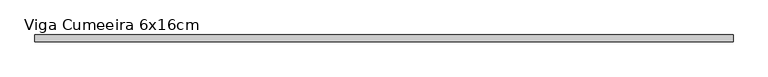
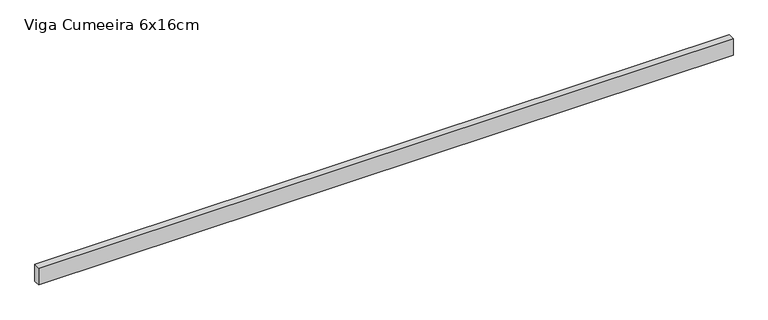
"""IFC4 building model written with IfcOpenShell, lengths in millimetres: beam geometry, Madeira de lei : Viga Cumeeira 6x16cm."""

from ifc_helpers import new_model, si_unit, frame, origin, place, context, project, spatial, polyline, outline, extrude, source, transform, mapped, element, save


def viga_cumeeira_6x16cm_e360fa9d(model_context):
    return source(origin(), model_context, "Body", "SweptSolid", [
        extrude(outline(polyline([(3133.5, 30.0), (3133.5, -30.0), (-3133.5, -30.0), (-3133.5, 30.0), (3133.5, 30.0)])), frame((0.0, 0.0, -80.0), z_axis=(0.0, 0.0, 1.0), x_axis=(1.0, 0.0, 0.0)), (0.0, 0.0, 1.0), 160.0),
    ])


if __name__ == "__main__":
    model = new_model("IFC4")
    model_context = context("Model", 3, world=origin())
    ifc_project = project(units=[si_unit("LENGTHUNIT", "METRE", prefix="MILLI")], contexts=[model_context])
    site = spatial("IfcSite", under=ifc_project)
    building = spatial("IfcBuilding", under=site)
    placement = place(None, origin())
    viga_cumeeira_6x16cm_shape = viga_cumeeira_6x16cm_e360fa9d(model_context)
    element("IfcBeam", 1, ObjectType="Madeira de lei : Viga Cumeeira 6x16cm", at=placement, inside=building, context=model_context, shape_type="MappedRepresentation", body=[
        mapped(viga_cumeeira_6x16cm_shape, transform((0.0, 0.0, 0.0), x_axis=(1.0, 0.0, 0.0), y_axis=(0.0, 1.0, 0.0), z_axis=(0.0, 0.0, 1.0))),
    ])
    save(model, "model.ifc")

# Revit data of these elements
# Type "Madeira de lei : Viga Cumeeira 6x16cm"
#   A = 0.02 m²
#   Length [instance default] = 1.524 m
#   b = 0.06 m
#   d = 0.16 m
#   Structural Material [instance default] = none
#   Assembly Code = ""
# Element 1 (IfcBeam, "Madeira de lei : Viga Cumeeira 6x16cm")
#   Structural Material = .MADEIRAMENTO
#   Materials on its faces: ".MADEIRAMENTO"
# Materials
#   ".MADEIRAMENTO": class ".CC_MADEIRAS", colour RGB 212 179 113, transparency 0, Cost = 0
